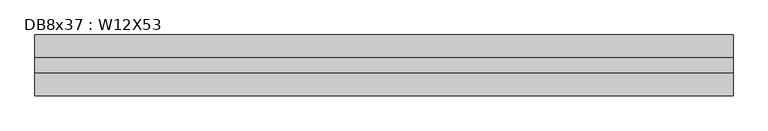
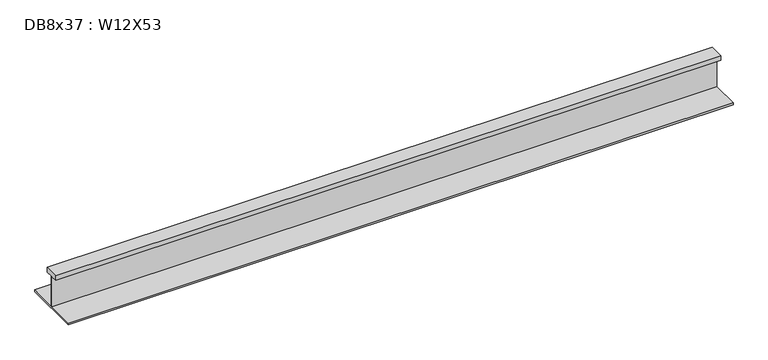
"""IFC4 building model written with IfcOpenShell, lengths in millimetres: beam geometry, DB8x37 : W12X53."""

from ifc_helpers import new_model, si_unit, frame, origin, place, context, project, spatial, polyline, outline, extrude, source, transform, mapped, element, save


def db8x37_w12x53_5a2d8ae1(model_context):
    return source(origin(), model_context, "Body", "SweptSolid", [
        extrude(outline(polyline([(38.1, 145.415), (38.1, 120.015), (2.921, 120.015), (2.921, -48.4505), (152.4, -48.4505), (152.4, -58.1025), (-152.4, -58.1025), (-152.4, -48.4505), (-2.921, -48.4505), (-2.921, 120.015), (-38.1, 120.015), (-38.1, 145.415), (38.1, 145.415)])), frame((-1699.6907198, 0.0, 0.0), z_axis=(1.0, 0.0, 0.0), x_axis=(0.0, 1.0, 0.0)), (0.0, 0.0, 1.0), 3500.6807508),
    ])


if __name__ == "__main__":
    model = new_model("IFC4")
    model_context = context("Model", 3, world=origin())
    ifc_project = project(units=[si_unit("LENGTHUNIT", "METRE", prefix="MILLI")], contexts=[model_context])
    site = spatial("IfcSite", under=ifc_project)
    building = spatial("IfcBuilding", under=site)
    placement = place(None, origin())
    db8x37_w12x53_shape = db8x37_w12x53_5a2d8ae1(model_context)
    element("IfcBeam", 1, ObjectType="DB8x37 : W12X53", at=placement, inside=building, context=model_context, shape_type="MappedRepresentation", body=[
        mapped(db8x37_w12x53_shape, transform((0.0, 0.0, 0.0), x_axis=(1.0, 0.0, 0.0), y_axis=(0.0, 1.0, 0.0), z_axis=(0.0, 0.0, 1.0))),
    ])
    save(model, "model.ifc")

# Revit data of these elements
# Type "DB8x37 : W12X53"
#   Assembly Code = "B10"
#   W = 53
#   Length [instance default] = 5' - 0"
#   bf = 0' - 10"
#   d = 1' - 0.1"
#   k = 0' - 1 3/8"
#   k2 = 0' - 0.8"
#   tf = 0' - 0.575"
#   tw = 0' - 0.345"
#   A = 0.108333 SF
#   Structural Material [instance default] = Steel ASTM A992
# Element 1 (IfcBeam, "DB8x37 : W12X53")
#   Materials on its faces: "Steel ASTM A992"
# Materials
#   "Steel ASTM A992": class "Metal", colour RGB 199 199 199, transparency 0, Description = "Structural steel 50ksi", Cost = 0
